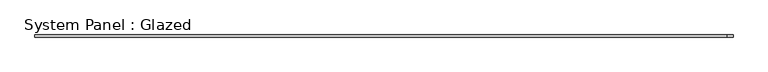
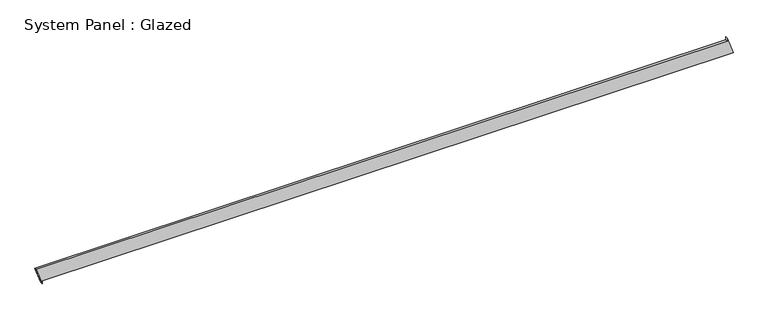
"""IFC4 building model written with IfcOpenShell, lengths in millimetres: plate geometry, System Panel : Glazed."""

from ifc_helpers import new_model, si_unit, frame, origin, place, context, project, spatial, polyline, outline, extrude, source, transform, mapped, element, save


def system_panel_glazed_d027619a(model_context):
    return source(origin(), model_context, "Body", "SweptSolid", [
        extrude(outline(polyline([(0.0, -3958.2331101), (35.3553391, -3958.2331101), (35.3553391, 4028.3015014), (235.2187437, 3958.3356687), (199.8634046, 3958.3358597), (199.8202529, -4028.3015014), (0.0, -3958.2331101)])), frame((0.0, -49.5, 0.0), z_axis=(0.0, 1.0, 0.0), x_axis=(0.0, 0.0, 1.0)), (0.0, 0.0, 1.0), 25.0),
    ])


if __name__ == "__main__":
    model = new_model("IFC4")
    model_context = context("Model", 3, world=origin())
    ifc_project = project(units=[si_unit("LENGTHUNIT", "METRE", prefix="MILLI")], contexts=[model_context])
    site = spatial("IfcSite", under=ifc_project)
    building = spatial("IfcBuilding", under=site)
    placement = place(None, origin())
    system_panel_glazed_shape = system_panel_glazed_d027619a(model_context)
    element("IfcPlate", 1, ObjectType="System Panel : Glazed", at=placement, inside=building, context=model_context, shape_type="MappedRepresentation", body=[
        mapped(system_panel_glazed_shape, transform((0.0, 0.0, 0.0), x_axis=(1.0, 0.0, 0.0), y_axis=(0.0, 1.0, 0.0), z_axis=(0.0, 0.0, 1.0))),
    ])
    save(model, "model.ifc")

# Revit data of these elements
# Element 1 (IfcPlate, "System Panel : Glazed")
#   Materials on its faces: "Glass"
# Materials
#   "Glass": class "Glass", colour RGB 218 227 224, transparency 0.85, Description = "Soda Lime Glass", Cost = 0
